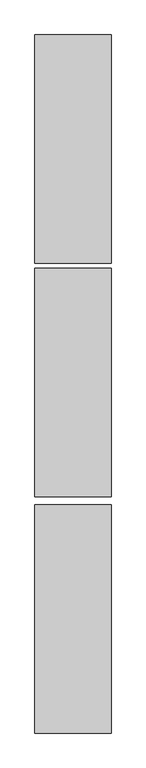
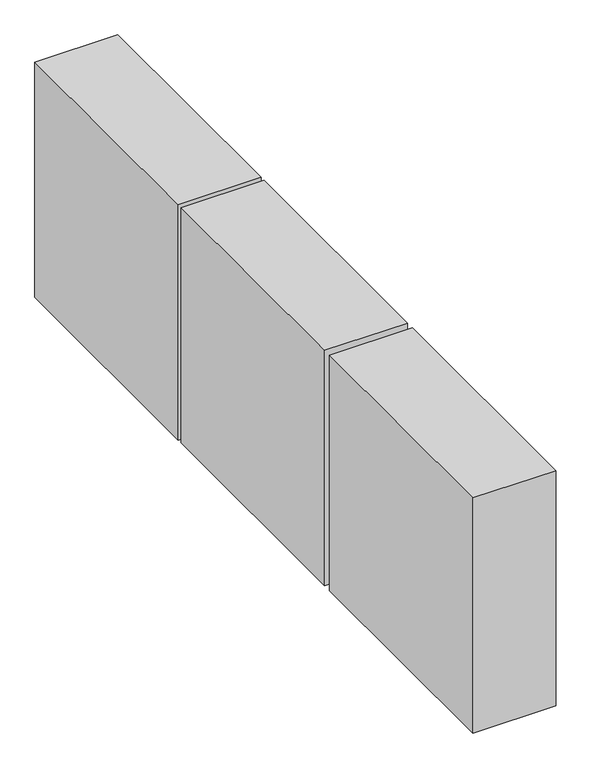
"""IFC4 building model written with IfcOpenShell, lengths in millimetres: furniture geometry, Metalic shelf : Metalic shelf."""

import ifcopenshell
import ifcopenshell.guid

model = None  # the IFC model being written
_history = None  # IfcOwnerHistory: only IFC2X3 demands one
_inside = {}  # id of a spatial element -> (the spatial element, [elements in it])
_under = {}  # id of a project, library or spatial element -> (it, [spatial elements below it])
_declared = {}  # id of a project -> (the project, [libraries it declares])
_typed = {}  # id of a type object -> (the type object, [elements of that type])
_made_of = {}  # id of a material, layer set ... -> (it, [elements and type objects made of it])


def new_model(schema):
    """Start an empty IFC model of exactly this schema.

    Asked for "IFC4X3", IfcOpenShell would pick the latest addendum, in which some entities
    have other attributes; the version numbers below select the first issue.
    IFC2X3 requires an IfcOwnerHistory on every rooted entity: one is made here for all.
    """
    global model, _history
    if schema == "IFC4X3":
        model = ifcopenshell.file(schema_version=(4, 3, 0, 0))
    else:
        model = ifcopenshell.file(schema=schema)
    _inside.clear()
    _under.clear()
    _declared.clear()
    _typed.clear()
    _made_of.clear()
    _history = None
    if model.schema == "IFC2X3":
        org = make("IfcOrganization", Name="unknown")
        user = make(
            "IfcPersonAndOrganization",
            ThePerson=make("IfcPerson", FamilyName="unknown"),
            TheOrganization=org,
        )
        app = make(
            "IfcApplication",
            ApplicationDeveloper=org,
            Version="unknown",
            ApplicationFullName="unknown",
            ApplicationIdentifier="unknown",
        )
        _history = make(
            "IfcOwnerHistory",
            OwningUser=user,
            OwningApplication=app,
            ChangeAction="ADDED",
            CreationDate=0,
        )
    return model


def make(cls, **values):
    """One entity of the class cls with the attributes given. An attribute that is None is left unset."""
    return model.create_entity(
        cls, **{name: value for name, value in values.items() if value is not None}
    )


def rooted(cls, **values):
    """An entity with a GlobalId (a new one), such as an element, a storey or a relation."""
    return make(cls, GlobalId=ifcopenshell.guid.new(), OwnerHistory=_history, **values)


def si_unit(unit_type, name, prefix=None):
    """IfcSIUnit, for example si_unit("LENGTHUNIT", "METRE", prefix="MILLI")."""
    return make("IfcSIUnit", UnitType=unit_type, Prefix=prefix, Name=name)


def assignment(units):
    """IfcUnitAssignment: the units of a project."""
    return None if units is None else make("IfcUnitAssignment", Units=units)


def point(xyz):
    """IfcCartesianPoint."""
    return None if xyz is None else make("IfcCartesianPoint", Coordinates=xyz)


def direction(xyz):
    """IfcDirection."""
    return None if xyz is None else make("IfcDirection", DirectionRatios=xyz)


def frame(location, z_axis=None, x_axis=None):
    """IfcAxis2Placement3D, a coordinate frame: its origin and axes. An axis left out is left unset."""
    return make(
        "IfcAxis2Placement3D",
        Location=point(location),
        Axis=direction(z_axis),
        RefDirection=direction(x_axis),
    )


def origin():
    """The frame at (0, 0, 0) with its axes left unset."""
    return frame((0.0, 0.0, 0.0))


def origin_with_axes():
    """The frame at (0, 0, 0) with the z axis (0, 0, 1) and the x axis (1, 0, 0) written out."""
    return frame((0.0, 0.0, 0.0), z_axis=(0.0, 0.0, 1.0), x_axis=(1.0, 0.0, 0.0))


def place(relative_to, where):
    """IfcLocalPlacement: puts the frame where relative to a parent placement (None: the world)."""
    return make(
        "IfcLocalPlacement", PlacementRelTo=relative_to, RelativePlacement=where
    )


def context(
    kind, dimensions, precision=None, world=None, true_north=None, identifier=None
):
    """IfcGeometricRepresentationContext, for example the 3D "Model" context."""
    return make(
        "IfcGeometricRepresentationContext",
        ContextIdentifier=identifier,
        ContextType=kind,
        CoordinateSpaceDimension=dimensions,
        Precision=precision,
        WorldCoordinateSystem=world,
        TrueNorth=true_north,
    )


def project(units=None, contexts=None):
    """IfcProject with its units and contexts."""
    return rooted(
        "IfcProject",
        Name="project",
        RepresentationContexts=contexts,
        UnitsInContext=assignment(units),
    )


def spatial(cls, under=None, at=None, **own):
    """A site, building, storey or space (cls), placed at a placement, below another one or the project."""
    s = rooted(cls, ObjectPlacement=at, **own)
    if under is not None:
        _under.setdefault(under.id(), (under, []))[1].append(s)
    return s


def polyline(points):
    """IfcPolyline through the points."""
    return make("IfcPolyline", Points=[point(p) for p in points])


def outline(outer, holes=None, kind="AREA"):
    """IfcArbitraryClosedProfileDef: a profile drawn as a closed curve; with holes, ...WithVoids."""
    if holes is None:
        return make("IfcArbitraryClosedProfileDef", ProfileType=kind, OuterCurve=outer)
    return make(
        "IfcArbitraryProfileDefWithVoids",
        ProfileType=kind,
        OuterCurve=outer,
        InnerCurves=holes,
    )


def extrude(swept, where, along, depth):
    """IfcExtrudedAreaSolid: the profile swept, set in the frame where, extruded along a direction by depth."""
    return make(
        "IfcExtrudedAreaSolid",
        SweptArea=swept,
        Position=where,
        ExtrudedDirection=direction(along),
        Depth=depth,
    )


def shape(context_of_items, identifier, shape_type, items):
    """IfcShapeRepresentation: the items that make up one representation, for example the "Body"."""
    return make(
        "IfcShapeRepresentation",
        ContextOfItems=context_of_items,
        RepresentationIdentifier=identifier,
        RepresentationType=shape_type,
        Items=items,
    )


def source(mapping_origin, context_of_items, identifier, shape_type, items):
    """IfcRepresentationMap: a shape defined once, which mapped items show again and again."""
    return make(
        "IfcRepresentationMap",
        MappingOrigin=mapping_origin,
        MappedRepresentation=shape(context_of_items, identifier, shape_type, items),
    )


def transform(
    local_origin,
    x_axis=None,
    y_axis=None,
    z_axis=None,
    scale=None,
    scale2=None,
    scale3=None,
    uniform=True,
):
    """IfcCartesianTransformationOperator3D, or its non-uniform kind. x_axis, y_axis, z_axis: its Axis1, 2, 3."""
    if uniform:
        return make(
            "IfcCartesianTransformationOperator3D",
            Axis1=direction(x_axis),
            Axis2=direction(y_axis),
            LocalOrigin=point(local_origin),
            Scale=scale,
            Axis3=direction(z_axis),
        )
    return make(
        "IfcCartesianTransformationOperator3DnonUniform",
        Axis1=direction(x_axis),
        Axis2=direction(y_axis),
        LocalOrigin=point(local_origin),
        Scale=scale,
        Axis3=direction(z_axis),
        Scale2=scale2,
        Scale3=scale3,
    )


def mapped(mapping_source, mapping_target):
    """IfcMappedItem: shows the shape of a source again, moved by a transform."""
    return make(
        "IfcMappedItem", MappingSource=mapping_source, MappingTarget=mapping_target
    )


def made_of(thing, what):
    """Note that an element or type object is made of a material, layer set ...; save() writes the relation."""
    if what is not None:
        _made_of.setdefault(what.id(), (what, []))[1].append(thing)
    return thing


def element(
    cls,
    number,
    at=None,
    inside=None,
    cuts=None,
    type_object=None,
    material=None,
    context=None,
    identifier="Body",
    shape_type=None,
    held_by="IfcProductDefinitionShape",
    body=None,
    shapes=None,
    **own,
):
    """One element of the class cls, such as IfcWall. Its Tag is "e" and its number.

    at: its placement. inside: the storey or other place that contains it. cuts: it is an
    opening in that element (IfcRelVoidsElement). A single representation is given by context,
    identifier, shape_type and body (its items); several are given by shapes. held_by: the class
    of the entity that holds the representations. save() writes the other relations.
    """
    e = rooted(cls, Tag="e%d" % number, ObjectPlacement=at, **own)
    if body is not None:
        shapes = [shape(context, identifier, shape_type, body)]
    if shapes is not None:
        e.Representation = make(held_by, Representations=shapes)
    if inside is not None:
        _inside.setdefault(inside.id(), (inside, []))[1].append(e)
    if cuts is not None:
        rooted(
            "IfcRelVoidsElement", RelatingBuildingElement=cuts, RelatedOpeningElement=e
        )
    if type_object is not None:
        _typed.setdefault(type_object.id(), (type_object, []))[1].append(e)
    return made_of(e, material)


def aggregate(whole, parts):
    """IfcRelAggregates: a whole, such as a stair, and the parts it consists of."""
    return rooted("IfcRelAggregates", RelatingObject=whole, RelatedObjects=parts)


def save(model, path):
    """Write the relations noted so far, then the file.

    IfcRelAggregates (storeys below a building ...), IfcRelContainedInSpatialStructure (elements
    in a storey), IfcRelDefinesByType, IfcRelAssociatesMaterial and IfcRelDeclares: one each for
    every whole, place, type object, material and project.
    """
    for whole, parts in _under.values():
        aggregate(whole, parts)
    for where, things in _inside.values():
        rooted(
            "IfcRelContainedInSpatialStructure",
            RelatedElements=things,
            RelatingStructure=where,
        )
    for kind, things in _typed.values():
        rooted("IfcRelDefinesByType", RelatedObjects=things, RelatingType=kind)
    for what, things in _made_of.values():
        rooted("IfcRelAssociatesMaterial", RelatedObjects=things, RelatingMaterial=what)
    for by, libraries in _declared.values():
        rooted("IfcRelDeclares", RelatingContext=by, RelatedDefinitions=libraries)
    model.write(path)


def furniture_fd3c48cc(model_context):
    return source(origin(), model_context, "Body", "SweptSolid", [
        extrude(outline(polyline([(24289.5370052, 4217.6615366), (23984.7370052, 4217.6615366), (23984.7370052, 5132.0615366), (24289.5370052, 5132.0615366), (24289.5370052, 4217.6615366)])), origin_with_axes(), (0.0, 0.0, 1.0), 914.4),
        extrude(outline(polyline([(24289.5370052, 3271.5115366), (23984.7370052, 3271.5115366), (23984.7370052, 4185.9115366), (24289.5370052, 4185.9115366), (24289.5370052, 3271.5115366)])), origin_with_axes(), (0.0, 0.0, 1.0), 914.4),
        extrude(outline(polyline([(24289.5370052, 5151.1115366), (23984.7370052, 5151.1115366), (23984.7370052, 6065.5115366), (24289.5370052, 6065.5115366), (24289.5370052, 5151.1115366)])), origin_with_axes(), (0.0, 0.0, 1.0), 914.4),
    ])


if __name__ == "__main__":
    model = new_model("IFC4")
    model_context = context("Model", 3, world=origin())
    ifc_project = project(units=[si_unit("LENGTHUNIT", "METRE", prefix="MILLI")], contexts=[model_context])
    site = spatial("IfcSite", under=ifc_project)
    building = spatial("IfcBuilding", under=site)
    placement = place(None, origin())
    furniture_shape = furniture_fd3c48cc(model_context)
    element("IfcFurniture", 1, ObjectType="Metalic shelf : Metalic shelf", at=placement, inside=building, context=model_context, shape_type="MappedRepresentation", body=[
        mapped(furniture_shape, transform((0.0, 0.0, 0.0), x_axis=(1.0, 0.0, 0.0), y_axis=(0.0, 1.0, 0.0), z_axis=(0.0, 0.0, 1.0))),
    ])
    save(model, "model.ifc")
